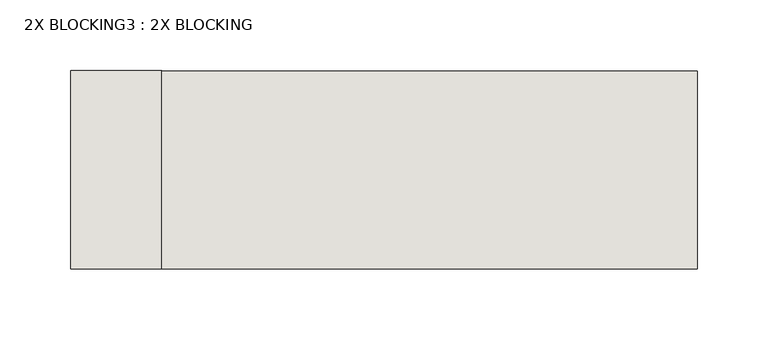
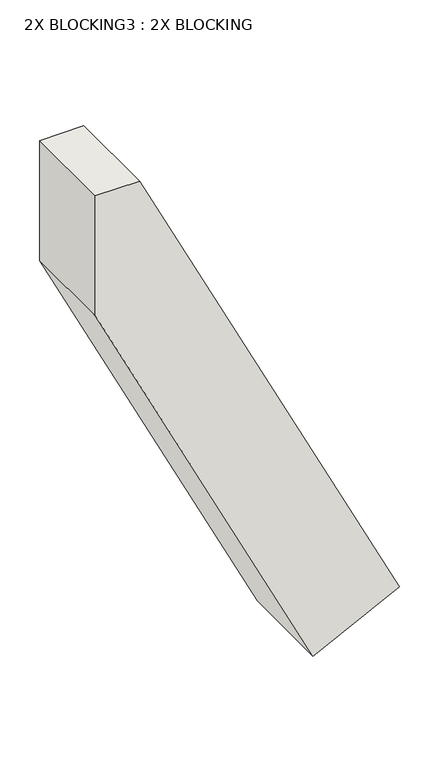
"""IFC4 building model written with IfcOpenShell, lengths in millimetres: wall geometry, 2X BLOCKING3 : 2X BLOCKING."""

from ifc_helpers import new_model, si_unit, frame, origin, place, context, project, spatial, polyline, outline, extrude, source, transform, mapped, element, save


def wall_2x_blocking3_2x_blocking_53facc28(model_context):
    return source(origin(), model_context, "Body", "SweptSolid", [
        extrude(outline(polyline([(4126.1923996, 23759.2172106), (4880.424114, 23382.1013534), (4880.424114, 23317.9870052), (4696.274114, 23317.9870052), (4063.7166603, 23634.265732), (4126.1923996, 23759.2172106)])), frame((0.0, -1256.0384634, 0.0), z_axis=(0.0, 1.0, 0.0), x_axis=(0.0, 0.0, 1.0)), (0.0, 0.0, 1.0), 139.7),
    ])


if __name__ == "__main__":
    model = new_model("IFC4")
    model_context = context("Model", 3, world=origin())
    ifc_project = project(units=[si_unit("LENGTHUNIT", "METRE", prefix="MILLI")], contexts=[model_context])
    site = spatial("IfcSite", under=ifc_project)
    building = spatial("IfcBuilding", under=site)
    placement = place(None, origin())
    wall_2x_blocking3_2x_blocking_shape = wall_2x_blocking3_2x_blocking_53facc28(model_context)
    element("IfcWall", 1, ObjectType="2X BLOCKING3 : 2X BLOCKING", at=placement, inside=building, context=model_context, shape_type="MappedRepresentation", body=[
        mapped(wall_2x_blocking3_2x_blocking_shape, transform((0.0, 0.0, 0.0), x_axis=(1.0, 0.0, 0.0), y_axis=(0.0, 1.0, 0.0), z_axis=(0.0, 0.0, 1.0))),
    ])
    save(model, "model.ifc")

# Revit data of these elements
# Type "2X BLOCKING3 : 2X BLOCKING"
#   Structural Material = 2 X BLOCKING
# Element 1 (IfcWall, "2X BLOCKING3 : 2X BLOCKING")
#   Materials on its faces: "2 X 6 RAFTER BEYOND"
# Materials
#   "2 X BLOCKING": class "Wood", colour RGB 234 198 147, transparency 0, Description = "Pinus Echinata", Cost = 0
#   "2 X 6 RAFTER BEYOND": class "Wood", colour RGB 234 198 147, transparency 0, Description = "Pinus Echinata", Cost = 0
